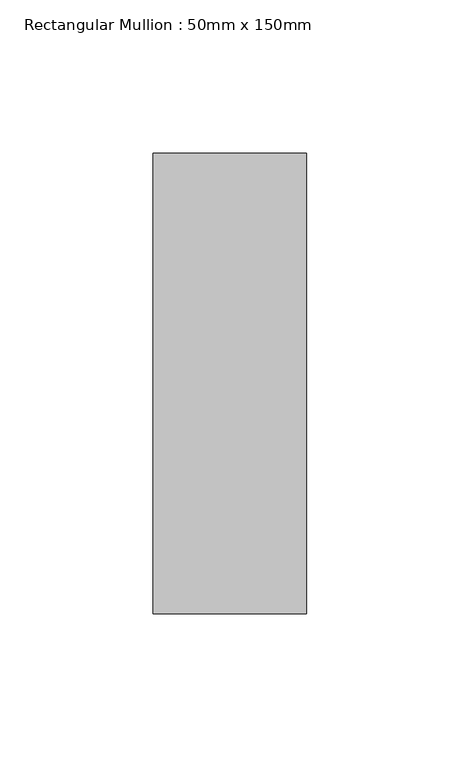
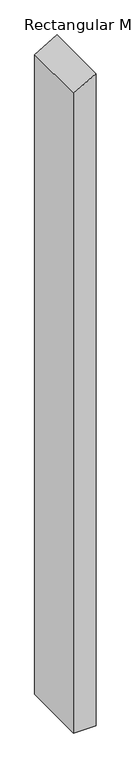
"""IFC4 building model written with IfcOpenShell, lengths in millimetres: member geometry, Rectangular Mullion : 50mm x 150mm."""

import ifcopenshell
import ifcopenshell.guid

model = None  # the IFC model being written
_history = None  # IfcOwnerHistory: only IFC2X3 demands one
_inside = {}  # id of a spatial element -> (the spatial element, [elements in it])
_under = {}  # id of a project, library or spatial element -> (it, [spatial elements below it])
_declared = {}  # id of a project -> (the project, [libraries it declares])
_typed = {}  # id of a type object -> (the type object, [elements of that type])
_made_of = {}  # id of a material, layer set ... -> (it, [elements and type objects made of it])


def new_model(schema):
    """Start an empty IFC model of exactly this schema.

    Asked for "IFC4X3", IfcOpenShell would pick the latest addendum, in which some entities
    have other attributes; the version numbers below select the first issue.
    IFC2X3 requires an IfcOwnerHistory on every rooted entity: one is made here for all.
    """
    global model, _history
    if schema == "IFC4X3":
        model = ifcopenshell.file(schema_version=(4, 3, 0, 0))
    else:
        model = ifcopenshell.file(schema=schema)
    _inside.clear()
    _under.clear()
    _declared.clear()
    _typed.clear()
    _made_of.clear()
    _history = None
    if model.schema == "IFC2X3":
        org = make("IfcOrganization", Name="unknown")
        user = make(
            "IfcPersonAndOrganization",
            ThePerson=make("IfcPerson", FamilyName="unknown"),
            TheOrganization=org,
        )
        app = make(
            "IfcApplication",
            ApplicationDeveloper=org,
            Version="unknown",
            ApplicationFullName="unknown",
            ApplicationIdentifier="unknown",
        )
        _history = make(
            "IfcOwnerHistory",
            OwningUser=user,
            OwningApplication=app,
            ChangeAction="ADDED",
            CreationDate=0,
        )
    return model


def make(cls, **values):
    """One entity of the class cls with the attributes given. An attribute that is None is left unset."""
    return model.create_entity(
        cls, **{name: value for name, value in values.items() if value is not None}
    )


def rooted(cls, **values):
    """An entity with a GlobalId (a new one), such as an element, a storey or a relation."""
    return make(cls, GlobalId=ifcopenshell.guid.new(), OwnerHistory=_history, **values)


def si_unit(unit_type, name, prefix=None):
    """IfcSIUnit, for example si_unit("LENGTHUNIT", "METRE", prefix="MILLI")."""
    return make("IfcSIUnit", UnitType=unit_type, Prefix=prefix, Name=name)


def assignment(units):
    """IfcUnitAssignment: the units of a project."""
    return None if units is None else make("IfcUnitAssignment", Units=units)


def point(xyz):
    """IfcCartesianPoint."""
    return None if xyz is None else make("IfcCartesianPoint", Coordinates=xyz)


def direction(xyz):
    """IfcDirection."""
    return None if xyz is None else make("IfcDirection", DirectionRatios=xyz)


def frame(location, z_axis=None, x_axis=None):
    """IfcAxis2Placement3D, a coordinate frame: its origin and axes. An axis left out is left unset."""
    return make(
        "IfcAxis2Placement3D",
        Location=point(location),
        Axis=direction(z_axis),
        RefDirection=direction(x_axis),
    )


def origin():
    """The frame at (0, 0, 0) with its axes left unset."""
    return frame((0.0, 0.0, 0.0))


def place(relative_to, where):
    """IfcLocalPlacement: puts the frame where relative to a parent placement (None: the world)."""
    return make(
        "IfcLocalPlacement", PlacementRelTo=relative_to, RelativePlacement=where
    )


def context(
    kind, dimensions, precision=None, world=None, true_north=None, identifier=None
):
    """IfcGeometricRepresentationContext, for example the 3D "Model" context."""
    return make(
        "IfcGeometricRepresentationContext",
        ContextIdentifier=identifier,
        ContextType=kind,
        CoordinateSpaceDimension=dimensions,
        Precision=precision,
        WorldCoordinateSystem=world,
        TrueNorth=true_north,
    )


def project(units=None, contexts=None):
    """IfcProject with its units and contexts."""
    return rooted(
        "IfcProject",
        Name="project",
        RepresentationContexts=contexts,
        UnitsInContext=assignment(units),
    )


def spatial(cls, under=None, at=None, **own):
    """A site, building, storey or space (cls), placed at a placement, below another one or the project."""
    s = rooted(cls, ObjectPlacement=at, **own)
    if under is not None:
        _under.setdefault(under.id(), (under, []))[1].append(s)
    return s


def polyline(points):
    """IfcPolyline through the points."""
    return make("IfcPolyline", Points=[point(p) for p in points])


def outline(outer, holes=None, kind="AREA"):
    """IfcArbitraryClosedProfileDef: a profile drawn as a closed curve; with holes, ...WithVoids."""
    if holes is None:
        return make("IfcArbitraryClosedProfileDef", ProfileType=kind, OuterCurve=outer)
    return make(
        "IfcArbitraryProfileDefWithVoids",
        ProfileType=kind,
        OuterCurve=outer,
        InnerCurves=holes,
    )


def extrude(swept, where, along, depth):
    """IfcExtrudedAreaSolid: the profile swept, set in the frame where, extruded along a direction by depth."""
    return make(
        "IfcExtrudedAreaSolid",
        SweptArea=swept,
        Position=where,
        ExtrudedDirection=direction(along),
        Depth=depth,
    )


def shape(context_of_items, identifier, shape_type, items):
    """IfcShapeRepresentation: the items that make up one representation, for example the "Body"."""
    return make(
        "IfcShapeRepresentation",
        ContextOfItems=context_of_items,
        RepresentationIdentifier=identifier,
        RepresentationType=shape_type,
        Items=items,
    )


def source(mapping_origin, context_of_items, identifier, shape_type, items):
    """IfcRepresentationMap: a shape defined once, which mapped items show again and again."""
    return make(
        "IfcRepresentationMap",
        MappingOrigin=mapping_origin,
        MappedRepresentation=shape(context_of_items, identifier, shape_type, items),
    )


def transform(
    local_origin,
    x_axis=None,
    y_axis=None,
    z_axis=None,
    scale=None,
    scale2=None,
    scale3=None,
    uniform=True,
):
    """IfcCartesianTransformationOperator3D, or its non-uniform kind. x_axis, y_axis, z_axis: its Axis1, 2, 3."""
    if uniform:
        return make(
            "IfcCartesianTransformationOperator3D",
            Axis1=direction(x_axis),
            Axis2=direction(y_axis),
            LocalOrigin=point(local_origin),
            Scale=scale,
            Axis3=direction(z_axis),
        )
    return make(
        "IfcCartesianTransformationOperator3DnonUniform",
        Axis1=direction(x_axis),
        Axis2=direction(y_axis),
        LocalOrigin=point(local_origin),
        Scale=scale,
        Axis3=direction(z_axis),
        Scale2=scale2,
        Scale3=scale3,
    )


def mapped(mapping_source, mapping_target):
    """IfcMappedItem: shows the shape of a source again, moved by a transform."""
    return make(
        "IfcMappedItem", MappingSource=mapping_source, MappingTarget=mapping_target
    )


def made_of(thing, what):
    """Note that an element or type object is made of a material, layer set ...; save() writes the relation."""
    if what is not None:
        _made_of.setdefault(what.id(), (what, []))[1].append(thing)
    return thing


def element(
    cls,
    number,
    at=None,
    inside=None,
    cuts=None,
    type_object=None,
    material=None,
    context=None,
    identifier="Body",
    shape_type=None,
    held_by="IfcProductDefinitionShape",
    body=None,
    shapes=None,
    **own,
):
    """One element of the class cls, such as IfcWall. Its Tag is "e" and its number.

    at: its placement. inside: the storey or other place that contains it. cuts: it is an
    opening in that element (IfcRelVoidsElement). A single representation is given by context,
    identifier, shape_type and body (its items); several are given by shapes. held_by: the class
    of the entity that holds the representations. save() writes the other relations.
    """
    e = rooted(cls, Tag="e%d" % number, ObjectPlacement=at, **own)
    if body is not None:
        shapes = [shape(context, identifier, shape_type, body)]
    if shapes is not None:
        e.Representation = make(held_by, Representations=shapes)
    if inside is not None:
        _inside.setdefault(inside.id(), (inside, []))[1].append(e)
    if cuts is not None:
        rooted(
            "IfcRelVoidsElement", RelatingBuildingElement=cuts, RelatedOpeningElement=e
        )
    if type_object is not None:
        _typed.setdefault(type_object.id(), (type_object, []))[1].append(e)
    return made_of(e, material)


def aggregate(whole, parts):
    """IfcRelAggregates: a whole, such as a stair, and the parts it consists of."""
    return rooted("IfcRelAggregates", RelatingObject=whole, RelatedObjects=parts)


def save(model, path):
    """Write the relations noted so far, then the file.

    IfcRelAggregates (storeys below a building ...), IfcRelContainedInSpatialStructure (elements
    in a storey), IfcRelDefinesByType, IfcRelAssociatesMaterial and IfcRelDeclares: one each for
    every whole, place, type object, material and project.
    """
    for whole, parts in _under.values():
        aggregate(whole, parts)
    for where, things in _inside.values():
        rooted(
            "IfcRelContainedInSpatialStructure",
            RelatedElements=things,
            RelatingStructure=where,
        )
    for kind, things in _typed.values():
        rooted("IfcRelDefinesByType", RelatedObjects=things, RelatingType=kind)
    for what, things in _made_of.values():
        rooted("IfcRelAssociatesMaterial", RelatedObjects=things, RelatingMaterial=what)
    for by, libraries in _declared.values():
        rooted("IfcRelDeclares", RelatingContext=by, RelatedDefinitions=libraries)
    model.write(path)


def rectangular_mullion_50mm_x_150mm_03c50f69(model_context):
    return source(origin(), model_context, "Body", "SweptSolid", [
        extrude(outline(polyline([(0.0, 0.0), (-28.8675135, -50.0), (-1534.1021441, -50.0), (-1534.1021441, 0.0), (0.0, 0.0)])), frame((0.0, -75.0, 0.0), z_axis=(0.0, 1.0, 0.0), x_axis=(0.0, 0.0, 1.0)), (0.0, 0.0, 1.0), 150.0),
    ])


if __name__ == "__main__":
    model = new_model("IFC4")
    model_context = context("Model", 3, world=origin())
    ifc_project = project(units=[si_unit("LENGTHUNIT", "METRE", prefix="MILLI")], contexts=[model_context])
    site = spatial("IfcSite", under=ifc_project)
    building = spatial("IfcBuilding", under=site)
    placement = place(None, origin())
    rectangular_mullion_50mm_x_150mm_shape = rectangular_mullion_50mm_x_150mm_03c50f69(model_context)
    element("IfcMember", 1, ObjectType="Rectangular Mullion : 50mm x 150mm", at=placement, inside=building, context=model_context, shape_type="MappedRepresentation", body=[
        mapped(rectangular_mullion_50mm_x_150mm_shape, transform((0.0, 0.0, 0.0), x_axis=(1.0, 0.0, 0.0), y_axis=(0.0, 1.0, 0.0), z_axis=(0.0, 0.0, 1.0))),
    ])
    save(model, "model.ifc")

# Revit data of these elements
# Type "Rectangular Mullion : 50mm x 150mm"
#   built-in parameter 1007304 = 0.492126 (stored number, unit not read)
#   built-in parameter 1007301 = 0.082021 (stored number, unit not read)
#   built-in parameter 1007300 = 0.082021 (stored number, unit not read)
# Element 1 (IfcMember, "Rectangular Mullion : 50mm x 150mm")
#   Materials on its faces: "Aluminum"
# Materials
#   "Aluminum": class "Metal", colour RGB 247 247 247, transparency 0, Description = "Aluminum 6061", Cost = 0
